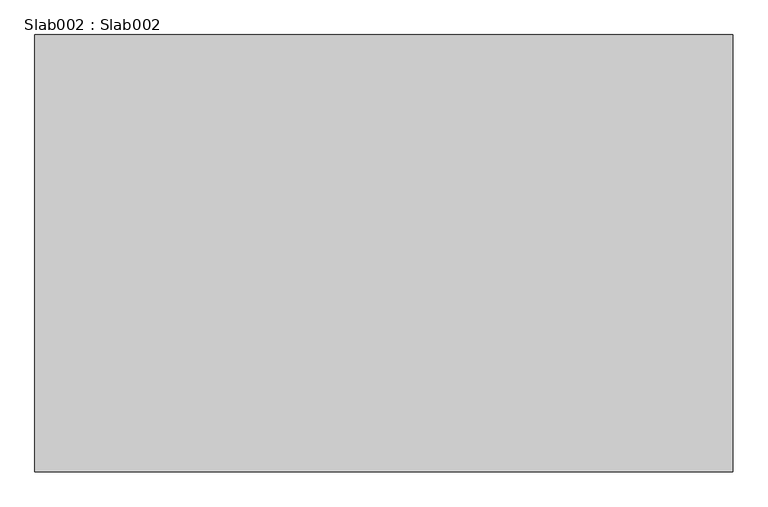
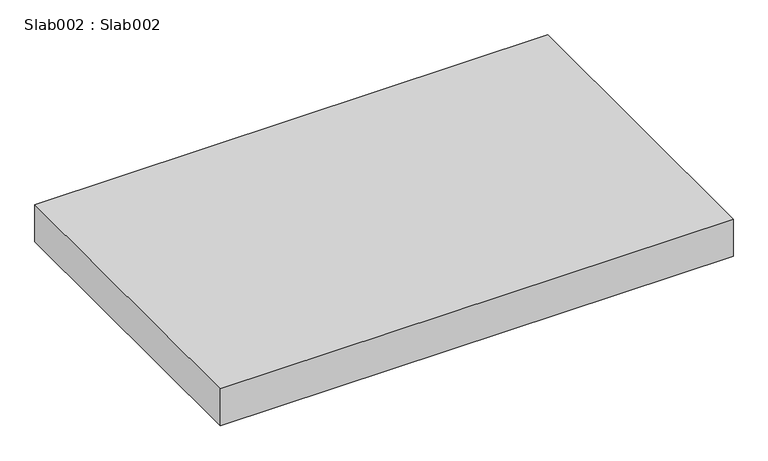
"""IFC4 building model written with IfcOpenShell, lengths in millimetres: proxy geometry, Slab002 : Slab002."""

import ifcopenshell
import ifcopenshell.guid

model = None  # the IFC model being written
_history = None  # IfcOwnerHistory: only IFC2X3 demands one
_inside = {}  # id of a spatial element -> (the spatial element, [elements in it])
_under = {}  # id of a project, library or spatial element -> (it, [spatial elements below it])
_declared = {}  # id of a project -> (the project, [libraries it declares])
_typed = {}  # id of a type object -> (the type object, [elements of that type])
_made_of = {}  # id of a material, layer set ... -> (it, [elements and type objects made of it])


def new_model(schema):
    """Start an empty IFC model of exactly this schema.

    Asked for "IFC4X3", IfcOpenShell would pick the latest addendum, in which some entities
    have other attributes; the version numbers below select the first issue.
    IFC2X3 requires an IfcOwnerHistory on every rooted entity: one is made here for all.
    """
    global model, _history
    if schema == "IFC4X3":
        model = ifcopenshell.file(schema_version=(4, 3, 0, 0))
    else:
        model = ifcopenshell.file(schema=schema)
    _inside.clear()
    _under.clear()
    _declared.clear()
    _typed.clear()
    _made_of.clear()
    _history = None
    if model.schema == "IFC2X3":
        org = make("IfcOrganization", Name="unknown")
        user = make(
            "IfcPersonAndOrganization",
            ThePerson=make("IfcPerson", FamilyName="unknown"),
            TheOrganization=org,
        )
        app = make(
            "IfcApplication",
            ApplicationDeveloper=org,
            Version="unknown",
            ApplicationFullName="unknown",
            ApplicationIdentifier="unknown",
        )
        _history = make(
            "IfcOwnerHistory",
            OwningUser=user,
            OwningApplication=app,
            ChangeAction="ADDED",
            CreationDate=0,
        )
    return model


def make(cls, **values):
    """One entity of the class cls with the attributes given. An attribute that is None is left unset."""
    return model.create_entity(
        cls, **{name: value for name, value in values.items() if value is not None}
    )


def rooted(cls, **values):
    """An entity with a GlobalId (a new one), such as an element, a storey or a relation."""
    return make(cls, GlobalId=ifcopenshell.guid.new(), OwnerHistory=_history, **values)


def si_unit(unit_type, name, prefix=None):
    """IfcSIUnit, for example si_unit("LENGTHUNIT", "METRE", prefix="MILLI")."""
    return make("IfcSIUnit", UnitType=unit_type, Prefix=prefix, Name=name)


def assignment(units):
    """IfcUnitAssignment: the units of a project."""
    return None if units is None else make("IfcUnitAssignment", Units=units)


def point(xyz):
    """IfcCartesianPoint."""
    return None if xyz is None else make("IfcCartesianPoint", Coordinates=xyz)


def direction(xyz):
    """IfcDirection."""
    return None if xyz is None else make("IfcDirection", DirectionRatios=xyz)


def frame(location, z_axis=None, x_axis=None):
    """IfcAxis2Placement3D, a coordinate frame: its origin and axes. An axis left out is left unset."""
    return make(
        "IfcAxis2Placement3D",
        Location=point(location),
        Axis=direction(z_axis),
        RefDirection=direction(x_axis),
    )


def origin():
    """The frame at (0, 0, 0) with its axes left unset."""
    return frame((0.0, 0.0, 0.0))


def place(relative_to, where):
    """IfcLocalPlacement: puts the frame where relative to a parent placement (None: the world)."""
    return make(
        "IfcLocalPlacement", PlacementRelTo=relative_to, RelativePlacement=where
    )


def context(
    kind, dimensions, precision=None, world=None, true_north=None, identifier=None
):
    """IfcGeometricRepresentationContext, for example the 3D "Model" context."""
    return make(
        "IfcGeometricRepresentationContext",
        ContextIdentifier=identifier,
        ContextType=kind,
        CoordinateSpaceDimension=dimensions,
        Precision=precision,
        WorldCoordinateSystem=world,
        TrueNorth=true_north,
    )


def project(units=None, contexts=None):
    """IfcProject with its units and contexts."""
    return rooted(
        "IfcProject",
        Name="project",
        RepresentationContexts=contexts,
        UnitsInContext=assignment(units),
    )


def spatial(cls, under=None, at=None, **own):
    """A site, building, storey or space (cls), placed at a placement, below another one or the project."""
    s = rooted(cls, ObjectPlacement=at, **own)
    if under is not None:
        _under.setdefault(under.id(), (under, []))[1].append(s)
    return s


def polyline(points):
    """IfcPolyline through the points."""
    return make("IfcPolyline", Points=[point(p) for p in points])


def outline(outer, holes=None, kind="AREA"):
    """IfcArbitraryClosedProfileDef: a profile drawn as a closed curve; with holes, ...WithVoids."""
    if holes is None:
        return make("IfcArbitraryClosedProfileDef", ProfileType=kind, OuterCurve=outer)
    return make(
        "IfcArbitraryProfileDefWithVoids",
        ProfileType=kind,
        OuterCurve=outer,
        InnerCurves=holes,
    )


def extrude(swept, where, along, depth):
    """IfcExtrudedAreaSolid: the profile swept, set in the frame where, extruded along a direction by depth."""
    return make(
        "IfcExtrudedAreaSolid",
        SweptArea=swept,
        Position=where,
        ExtrudedDirection=direction(along),
        Depth=depth,
    )


def shape(context_of_items, identifier, shape_type, items):
    """IfcShapeRepresentation: the items that make up one representation, for example the "Body"."""
    return make(
        "IfcShapeRepresentation",
        ContextOfItems=context_of_items,
        RepresentationIdentifier=identifier,
        RepresentationType=shape_type,
        Items=items,
    )


def source(mapping_origin, context_of_items, identifier, shape_type, items):
    """IfcRepresentationMap: a shape defined once, which mapped items show again and again."""
    return make(
        "IfcRepresentationMap",
        MappingOrigin=mapping_origin,
        MappedRepresentation=shape(context_of_items, identifier, shape_type, items),
    )


def transform(
    local_origin,
    x_axis=None,
    y_axis=None,
    z_axis=None,
    scale=None,
    scale2=None,
    scale3=None,
    uniform=True,
):
    """IfcCartesianTransformationOperator3D, or its non-uniform kind. x_axis, y_axis, z_axis: its Axis1, 2, 3."""
    if uniform:
        return make(
            "IfcCartesianTransformationOperator3D",
            Axis1=direction(x_axis),
            Axis2=direction(y_axis),
            LocalOrigin=point(local_origin),
            Scale=scale,
            Axis3=direction(z_axis),
        )
    return make(
        "IfcCartesianTransformationOperator3DnonUniform",
        Axis1=direction(x_axis),
        Axis2=direction(y_axis),
        LocalOrigin=point(local_origin),
        Scale=scale,
        Axis3=direction(z_axis),
        Scale2=scale2,
        Scale3=scale3,
    )


def mapped(mapping_source, mapping_target):
    """IfcMappedItem: shows the shape of a source again, moved by a transform."""
    return make(
        "IfcMappedItem", MappingSource=mapping_source, MappingTarget=mapping_target
    )


def made_of(thing, what):
    """Note that an element or type object is made of a material, layer set ...; save() writes the relation."""
    if what is not None:
        _made_of.setdefault(what.id(), (what, []))[1].append(thing)
    return thing


def element(
    cls,
    number,
    at=None,
    inside=None,
    cuts=None,
    type_object=None,
    material=None,
    context=None,
    identifier="Body",
    shape_type=None,
    held_by="IfcProductDefinitionShape",
    body=None,
    shapes=None,
    **own,
):
    """One element of the class cls, such as IfcWall. Its Tag is "e" and its number.

    at: its placement. inside: the storey or other place that contains it. cuts: it is an
    opening in that element (IfcRelVoidsElement). A single representation is given by context,
    identifier, shape_type and body (its items); several are given by shapes. held_by: the class
    of the entity that holds the representations. save() writes the other relations.
    """
    e = rooted(cls, Tag="e%d" % number, ObjectPlacement=at, **own)
    if body is not None:
        shapes = [shape(context, identifier, shape_type, body)]
    if shapes is not None:
        e.Representation = make(held_by, Representations=shapes)
    if inside is not None:
        _inside.setdefault(inside.id(), (inside, []))[1].append(e)
    if cuts is not None:
        rooted(
            "IfcRelVoidsElement", RelatingBuildingElement=cuts, RelatedOpeningElement=e
        )
    if type_object is not None:
        _typed.setdefault(type_object.id(), (type_object, []))[1].append(e)
    return made_of(e, material)


def aggregate(whole, parts):
    """IfcRelAggregates: a whole, such as a stair, and the parts it consists of."""
    return rooted("IfcRelAggregates", RelatingObject=whole, RelatedObjects=parts)


def save(model, path):
    """Write the relations noted so far, then the file.

    IfcRelAggregates (storeys below a building ...), IfcRelContainedInSpatialStructure (elements
    in a storey), IfcRelDefinesByType, IfcRelAssociatesMaterial and IfcRelDeclares: one each for
    every whole, place, type object, material and project.
    """
    for whole, parts in _under.values():
        aggregate(whole, parts)
    for where, things in _inside.values():
        rooted(
            "IfcRelContainedInSpatialStructure",
            RelatedElements=things,
            RelatingStructure=where,
        )
    for kind, things in _typed.values():
        rooted("IfcRelDefinesByType", RelatedObjects=things, RelatingType=kind)
    for what, things in _made_of.values():
        rooted("IfcRelAssociatesMaterial", RelatedObjects=things, RelatingMaterial=what)
    for by, libraries in _declared.values():
        rooted("IfcRelDeclares", RelatingContext=by, RelatedDefinitions=libraries)
    model.write(path)


def slab002_slab002_b16c44ad(model_context):
    return source(origin(), model_context, "Body", "SweptSolid", [
        extrude(outline(polyline([(14383.0178845, -4651.5044925), (14383.0178845, -5904.2981766), (12383.0178845, -5904.2981766), (12383.0178845, -4651.5044925), (14383.0178845, -4651.5044925)])), frame((0.0, 0.0, 36175.6882407), z_axis=(0.0, 0.0, 1.0), x_axis=(1.0, 0.0, 0.0)), (0.0, 0.0, 1.0), 152.4077593),
    ])


if __name__ == "__main__":
    model = new_model("IFC4")
    model_context = context("Model", 3, world=origin())
    ifc_project = project(units=[si_unit("LENGTHUNIT", "METRE", prefix="MILLI")], contexts=[model_context])
    site = spatial("IfcSite", under=ifc_project)
    building = spatial("IfcBuilding", under=site)
    placement = place(None, origin())
    slab002_slab002_shape = slab002_slab002_b16c44ad(model_context)
    element("IfcBuildingElementProxy", 1, Name="Slab002 : Slab002", ObjectType="Slab002 : Slab002", at=placement, inside=building, context=model_context, shape_type="MappedRepresentation", body=[
        mapped(slab002_slab002_shape, transform((0.0, 0.0, 0.0), x_axis=(1.0, 0.0, 0.0), y_axis=(0.0, 1.0, 0.0), z_axis=(0.0, 0.0, 1.0))),
    ])
    save(model, "model.ifc")

# Revit data of these elements
# Type "Slab002 : Slab002"
#   NameOverride = "Slab002"
# Element 1 (IfcBuildingElementProxy, "Slab002 : Slab002")
#   Materials on its faces: "4\" CONCRETE SLAB - SEE CIVIL DWGS"
# Materials
#   "4\" CONCRETE SLAB - SEE CIVIL DWGS": class "Unassigned", colour RGB 128 128 128, transparency 0, Cost = 0
